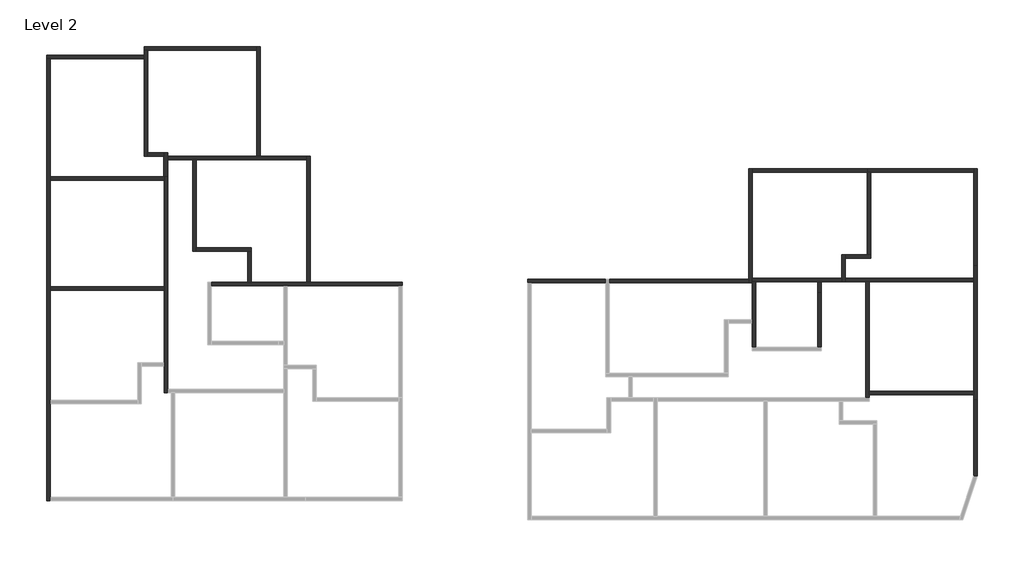
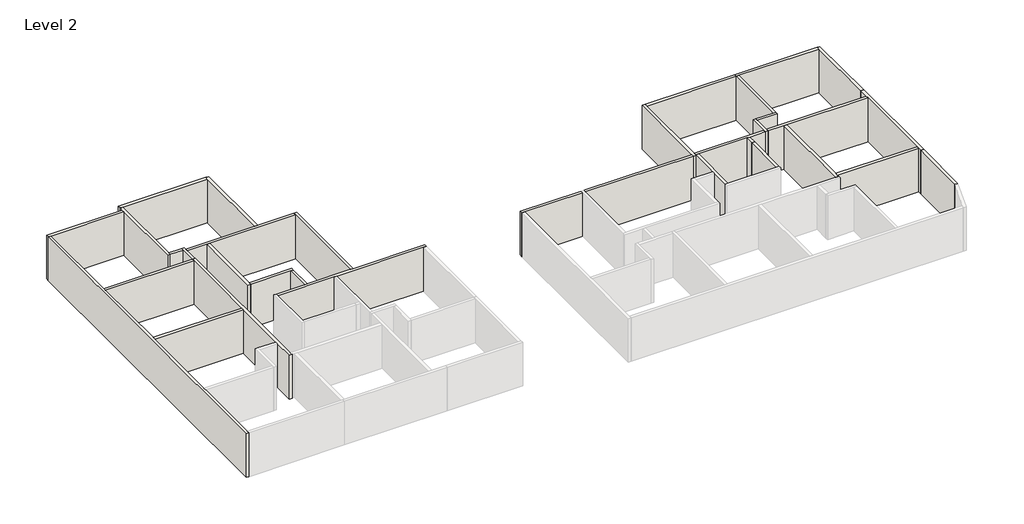
# One storey, part 2 of 2: 34 walls.
"""IFC4 building model written with IfcOpenShell, lengths in millimetres."""

from ifc_helpers import new_model, si_unit, frame, origin, place, context, project, spatial, polyline, outline, extrude, faceted_brep, element, save

model = new_model("IFC4")

# Units and contexts
model_context = context("Model", 3, world=origin())
ifc_project = project(units=[si_unit("LENGTHUNIT", "METRE", prefix="MILLI")], contexts=[model_context])

# Site, building, storey
site = spatial("IfcSite", under=ifc_project)
building = spatial("IfcBuilding", under=site)
storey = spatial("IfcBuildingStorey", under=building, Name="Level 2", Elevation=3000.0)

# Walls
placement = place(None, origin())
element("IfcWall", 1, ObjectType="Generic - 200mm", at=placement, inside=storey, context=model_context, shape_type="Brep", body=[
    faceted_brep([(24049.836337, 7619.475628, 3000.0), (24249.836337, 7619.475628, 3000.0), (30068.3425199, 7619.475628, 3000.0), (30068.3425199, 7619.475628, 6360.0), (24249.836337, 7619.475628, 6360.0), (24049.836337, 7619.475628, 6360.0), (24049.836337, 7819.475628, 3000.0), (24049.836337, 7819.475628, 6360.0), (30068.3425199, 7819.475628, 6360.0), (30068.3425199, 7819.475628, 3000.0)], [[[0, 1, 2, 3, 4, 5]], [[6, 7, 8, 9]], [[2, 1, 0, 6, 9]], [[5, 4, 3, 8, 7]], [[3, 2, 9, 8]], [[0, 5, 7, 6]]]),
])
element("IfcWall", 2, ObjectType="Generic - 200mm", at=placement, inside=storey, context=model_context, shape_type="Brep", body=[
    faceted_brep([(30068.3425199, 7819.475628, 3000.0), (30068.3425199, 7619.475628, 3000.0), (30068.3425199, 2319.475628, 3000.0), (30068.3425199, 2319.475628, 6360.0), (30068.3425199, 7619.475628, 6360.0), (30068.3425199, 7819.475628, 6360.0), (30268.3425199, 7819.475628, 3000.0), (30268.3425199, 7819.475628, 6360.0), (30268.3425199, 2319.475628, 6360.0), (30268.3425199, 2319.475628, 3000.0), (30117.9969803, 2319.475628, 3000.0), (30068.8612349, 2319.475628, 3000.0), (30068.8612349, 2319.475628, 6360.0)], [[[0, 1, 2, 3, 4, 5]], [[6, 7, 8, 9]], [[2, 1, 0, 6, 9, 10, 11]], [[3, 2, 11, 10, 9, 8, 12]], [[5, 4, 3, 12, 8, 7]], [[0, 5, 7, 6]]]),
])
element("IfcWall", 3, ObjectType="Generic - 200mm", at=placement, inside=storey, context=model_context, shape_type="Brep", body=[
    faceted_brep([(30068.8612349, 2319.475628, 3000.0), (30068.8612349, 1619.475628, 3000.0), (30068.8612349, 1419.475628, 3000.0), (30068.8612349, -4760.0098119, 3000.0), (30068.8612349, -4960.0098119, 3000.0), (30068.8612349, -5240.0098119, 3000.0), (30068.8612349, -5240.0098119, 6360.0), (30068.8612349, -4960.0098119, 6360.0), (30068.8612349, -4760.0098119, 6360.0), (30068.8612349, 1419.475628, 6360.0), (30068.8612349, 1619.475628, 6360.0), (30068.8612349, 2319.475628, 6360.0), (30268.8612349, 2319.475628, 3000.0), (30268.8612349, 2319.475628, 6360.0), (30268.8612349, -5240.0098119, 6360.0), (30268.8612349, -5240.0098119, 3000.0), (30118.5156953, 2319.475628, 3000.0), (30268.3425199, 2319.475628, 3000.0), (30118.5156953, -5240.0098119, 3000.0), (30069.3799498, -5240.0098119, 3000.0), (30069.3799498, -5240.0098119, 6360.0), (30268.3425199, 2319.475628, 6360.0)], [[[0, 1, 2, 3, 4, 5, 6, 7, 8, 9, 10, 11]], [[12, 13, 14, 15]], [[5, 4, 3, 2, 1, 0, 16, 17, 12, 15, 18, 19]], [[6, 5, 19, 18, 15, 14, 20]], [[11, 10, 9, 8, 7, 6, 20, 14, 13, 21]], [[0, 11, 21, 13, 12, 17, 16]]]),
])
element("IfcWall", 4, ObjectType="Generic - 200mm", at=placement, inside=storey, context=model_context, shape_type="Brep", body=[
    faceted_brep([(30069.3799498, -5240.0098119, 3000.0), (30069.3799498, -9543.0251929, 3000.0), (30069.3799498, -9543.0251929, 6360.0), (30069.3799498, -5240.0098119, 6360.0), (30269.3799498, -5240.0098119, 3000.0), (30269.3799498, -5240.0098119, 6360.0), (30269.3799498, -9575.863443, 6360.0), (30269.3799498, -9575.863443, 3000.0), (30119.0344102, -5240.0098119, 3000.0), (30268.8612349, -5240.0098119, 3000.0), (30268.8612349, -5240.0098119, 6360.0)], [[[0, 1, 2, 3]], [[4, 5, 6, 7]], [[1, 0, 8, 9, 4, 7]], [[3, 2, 6, 5, 10]], [[0, 3, 10, 5, 4, 9, 8]], [[2, 1, 7, 6]]]),
])
element("IfcWall", 5, ObjectType="Generic - 200mm", at=placement, inside=storey, context=model_context, shape_type="Brep", body=[
    faceted_brep([(24148.8612349, -5140.0098119, 3000.0), (24148.8612349, -4960.0098119, 3000.0), (24148.8612349, -4760.0098119, 3000.0), (24148.8612349, 1419.475628, 3000.0), (24148.8612349, 1419.475628, 6360.0), (24148.8612349, -4760.0098119, 6360.0), (24148.8612349, -4960.0098119, 6360.0), (24148.8612349, -5140.0098119, 6360.0), (23948.8612349, -5140.0098119, 3000.0), (23948.8612349, -5140.0098119, 6360.0), (23948.8612349, 1419.475628, 6360.0), (23948.8612349, 1419.475628, 3000.0)], [[[0, 1, 2, 3, 4, 5, 6, 7]], [[8, 9, 10, 11]], [[3, 2, 1, 0, 8, 11]], [[7, 6, 5, 4, 10, 9]], [[4, 3, 11, 10]], [[0, 7, 9, 8]]]),
])
element("IfcWall", 6, ObjectType="Generic - 200mm", at=placement, inside=storey, context=model_context, shape_type="Brep", body=[
    faceted_brep([(21249.836337, 799.475628, 3000.0), (21249.836337, -2276.2808257, 3000.0), (21249.836337, -2276.2808257, 6360.0), (21249.836337, 799.475628, 6360.0), (21449.836337, 799.475628, 3000.0), (21449.836337, 799.475628, 6360.0), (21449.836337, -2276.2808257, 6360.0), (21449.836337, -2276.2808257, 3000.0), (21299.4907974, 799.475628, 3000.0)], [[[0, 1, 2, 3]], [[4, 5, 6, 7]], [[1, 0, 8, 4, 7]], [[3, 2, 6, 5]], [[0, 3, 5, 4, 8]], [[2, 1, 7, 6]]]),
])
element("IfcWall", 7, ObjectType="Generic - 200mm", at=placement, inside=storey, context=model_context, shape_type="Brep", body=[
    faceted_brep([(17530.6041014, 1419.475628, 3000.0), (17530.6041014, -720.524372, 3000.0), (17530.6041014, -920.524372, 3000.0), (17530.6041014, -2276.2808257, 3000.0), (17530.6041014, -2276.2808257, 6360.0), (17530.6041014, -920.524372, 6360.0), (17530.6041014, -720.524372, 6360.0), (17530.6041014, 1419.475628, 6360.0), (17730.6041014, 1419.475628, 3000.0), (17730.6041014, 1419.475628, 6360.0), (17730.6041014, -2276.2808257, 6360.0), (17730.6041014, -2276.2808257, 3000.0)], [[[0, 1, 2, 3, 4, 5, 6, 7]], [[8, 9, 10, 11]], [[3, 2, 1, 0, 8, 11]], [[7, 6, 5, 4, 10, 9]], [[4, 3, 11, 10]], [[0, 7, 9, 8]]]),
])
element("IfcWall", 8, ObjectType="Generic - 200mm", at=placement, inside=storey, context=model_context, shape_type="Brep", body=[
    faceted_brep([(21449.836337, 799.475628, 3000.0), (21449.836337, 1419.475628, 3000.0), (21449.836337, 1419.475628, 6360.0), (21449.836337, 799.475628, 6360.0), (21249.836337, 799.475628, 3000.0), (21249.836337, 799.475628, 6360.0), (21249.836337, 1419.475628, 6360.0), (21249.836337, 1419.475628, 3000.0), (21299.4907974, 799.475628, 3000.0)], [[[0, 1, 2, 3]], [[4, 5, 6, 7]], [[1, 0, 8, 4, 7]], [[3, 2, 6, 5]], [[0, 3, 5, 4, 8]], [[2, 1, 7, 6]]]),
])
element("IfcWall", 9, ObjectType="Generic - 200mm", at=placement, inside=storey, context=model_context, shape_type="SweptSolid", body=[
    extrude(outline(polyline([(24049.836337, 7619.475628), (17528.8612349, 7619.475628), (17528.8612349, 7819.475628), (24049.836337, 7819.475628), (24049.836337, 7619.475628)])), frame((0.0, 0.0, 3000.0), z_axis=(0.0, 0.0, 1.0), x_axis=(1.0, 0.0, 0.0)), (0.0, 0.0, 1.0), 3360.0),
])
element("IfcWall", 10, ObjectType="Generic - 200mm", at=placement, inside=storey, context=model_context, shape_type="Brep", body=[
    faceted_brep([(22789.836337, 1419.475628, 3000.0), (22789.836337, 1619.475628, 3000.0), (22789.836337, 2754.475628, 3000.0), (22789.836337, 2954.475628, 3000.0), (22789.836337, 2954.475628, 6360.0), (22789.836337, 2754.475628, 6360.0), (22789.836337, 1619.475628, 6360.0), (22789.836337, 1419.475628, 6360.0), (22589.836337, 1419.475628, 3000.0), (22589.836337, 1419.475628, 6360.0), (22589.836337, 1619.475628, 6360.0), (22589.836337, 2954.475628, 6360.0), (22589.836337, 2954.475628, 3000.0), (22589.836337, 1619.475628, 3000.0)], [[[0, 1, 2, 3, 4, 5, 6, 7]], [[8, 9, 10, 11, 12, 13]], [[3, 2, 1, 0, 8, 13, 12]], [[7, 6, 5, 4, 11, 10, 9]], [[0, 7, 9, 8]], [[4, 3, 12, 11]]]),
])
element("IfcWall", 11, ObjectType="Generic - 200mm", at=placement, inside=storey, context=model_context, shape_type="Brep", body=[
    faceted_brep([(17328.8612349, 7819.475628, 3000.0), (17328.8612349, 1579.475628, 3000.0), (17328.8612349, 1379.475628, 3000.0), (17328.8612349, 1379.475628, 6360.0), (17328.8612349, 1579.475628, 6360.0), (17328.8612349, 7819.475628, 6360.0), (17528.8612349, 7819.475628, 3000.0), (17528.8612349, 7819.475628, 6360.0), (17528.8612349, 7619.475628, 6360.0), (17528.8612349, 1619.475628, 6360.0), (17528.8612349, 1419.475628, 6360.0), (17528.8612349, 1379.475628, 6360.0), (17528.8612349, 1379.475628, 3000.0), (17528.8612349, 1419.475628, 3000.0), (17528.8612349, 1619.475628, 3000.0), (17528.8612349, 7619.475628, 3000.0)], [[[0, 1, 2, 3, 4, 5]], [[6, 7, 8, 9, 10, 11, 12, 13, 14, 15]], [[2, 1, 0, 6, 15, 14, 13, 12]], [[5, 4, 3, 11, 10, 9, 8, 7]], [[0, 5, 7, 6]], [[3, 2, 12, 11]]]),
])
element("IfcWall", 12, ObjectType="Generic - 200mm", at=placement, inside=storey, context=model_context, shape_type="Brep", body=[
    faceted_brep([(22789.836337, 1419.475628, 3000.0), (23948.8612349, 1419.475628, 3000.0), (24148.8612349, 1419.475628, 3000.0), (30068.8612349, 1419.475628, 3000.0), (30068.8612349, 1419.475628, 6360.0), (24148.8612349, 1419.475628, 6360.0), (23948.8612349, 1419.475628, 6360.0), (22789.836337, 1419.475628, 6360.0), (22789.836337, 1619.475628, 3000.0), (22789.836337, 1619.475628, 6360.0), (30068.8612349, 1619.475628, 6360.0), (30068.8612349, 1619.475628, 3000.0)], [[[0, 1, 2, 3, 4, 5, 6, 7]], [[8, 9, 10, 11]], [[3, 2, 1, 0, 8, 11]], [[7, 6, 5, 4, 10, 9]], [[4, 3, 11, 10]], [[0, 7, 9, 8]]]),
])
element("IfcWall", 13, ObjectType="Generic - 200mm", at=placement, inside=storey, context=model_context, shape_type="SweptSolid", body=[
    extrude(outline(polyline([(9468.8612349, 1579.475628), (17328.8612349, 1579.475628), (17328.8612349, 1379.475628), (9468.8612349, 1379.475628), (9468.8612349, 1579.475628)])), frame((0.0, 0.0, 3000.0), z_axis=(0.0, 0.0, 1.0), x_axis=(1.0, 0.0, 0.0)), (0.0, 0.0, 1.0), 3360.0),
])
element("IfcWall", 14, ObjectType="Generic - 200mm", at=placement, inside=storey, context=model_context, shape_type="Brep", body=[
    faceted_brep([(22589.836337, 1619.475628, 3000.0), (17528.8612349, 1619.475628, 3000.0), (17528.8612349, 1619.475628, 6360.0), (22589.836337, 1619.475628, 6360.0), (22589.836337, 1419.475628, 3000.0), (22589.836337, 1419.475628, 6360.0), (21449.836337, 1419.475628, 6360.0), (21249.836337, 1419.475628, 6360.0), (17730.6041014, 1419.475628, 6360.0), (17530.6041014, 1419.475628, 6360.0), (17528.8612349, 1419.475628, 6360.0), (17528.8612349, 1419.475628, 3000.0), (17530.6041014, 1419.475628, 3000.0), (17730.6041014, 1419.475628, 3000.0), (21249.836337, 1419.475628, 3000.0), (21449.836337, 1419.475628, 3000.0)], [[[0, 1, 2, 3]], [[4, 5, 6, 7, 8, 9, 10, 11, 12, 13, 14, 15]], [[1, 0, 4, 15, 14, 13, 12, 11]], [[3, 2, 10, 9, 8, 7, 6, 5]], [[0, 3, 5, 4]], [[2, 1, 11, 10]]]),
])
element("IfcWall", 15, ObjectType="Generic - 200mm", at=placement, inside=storey, context=model_context, shape_type="Brep", body=[
    faceted_brep([(22789.836337, 2754.475628, 3000.0), (24249.836337, 2754.475628, 3000.0), (24249.836337, 2754.475628, 6360.0), (22789.836337, 2754.475628, 6360.0), (22789.836337, 2954.475628, 3000.0), (22789.836337, 2954.475628, 6360.0), (24049.836337, 2954.475628, 6360.0), (24249.836337, 2954.475628, 6360.0), (24249.836337, 2954.475628, 3000.0), (24049.836337, 2954.475628, 3000.0)], [[[0, 1, 2, 3]], [[4, 5, 6, 7, 8, 9]], [[1, 0, 4, 9, 8]], [[3, 2, 7, 6, 5]], [[2, 1, 8, 7]], [[0, 3, 5, 4]]]),
])
element("IfcWall", 16, ObjectType="Generic - 200mm", at=placement, inside=storey, context=model_context, shape_type="SweptSolid", body=[
    extrude(outline(polyline([(24249.836337, 7619.475628), (24249.836337, 2954.475628), (24049.836337, 2954.475628), (24049.836337, 7619.475628), (24249.836337, 7619.475628)])), frame((0.0, 0.0, 3000.0), z_axis=(0.0, 0.0, 1.0), x_axis=(1.0, 0.0, 0.0)), (0.0, 0.0, 1.0), 3360.0),
])
element("IfcWall", 17, ObjectType="Generic - 200mm", at=placement, inside=storey, context=model_context, shape_type="SweptSolid", body=[
    extrude(outline(polyline([(30068.8612349, -4960.0098119), (24148.8612349, -4960.0098119), (24148.8612349, -4760.0098119), (30068.8612349, -4760.0098119), (30068.8612349, -4960.0098119)])), frame((0.0, 0.0, 3000.0), z_axis=(0.0, 0.0, 1.0), x_axis=(1.0, 0.0, 0.0)), (0.0, 0.0, 1.0), 3360.0),
])
element("IfcWall", 18, ObjectType="Generic - 200mm", at=placement, inside=storey, context=model_context, shape_type="SweptSolid", body=[
    extrude(outline(polyline([(-15689.8304233, 949.8621849), (-22146.5113948, 949.8621849), (-22146.5113948, 1149.8621849), (-15689.8304233, 1149.8621849), (-15689.8304233, 949.8621849)])), frame((0.0, 0.0, 3000.0), z_axis=(0.0, 0.0, 1.0), x_axis=(1.0, 0.0, 0.0)), (0.0, 0.0, 1.0), 3360.0),
])
element("IfcWall", 19, ObjectType="Generic - 200mm", at=placement, inside=storey, context=model_context, shape_type="Brep", body=[
    faceted_brep([(-22146.5113948, -10959.6814279, 3000.0), (-22146.5113948, -10759.6814279, 3000.0), (-22146.5113948, -5479.1627129, 3000.0), (-22146.5113948, -5279.1627129, 3000.0), (-22146.5113948, 949.8621849, 3000.0), (-22146.5113948, 1149.8621849, 3000.0), (-22146.5113948, 7149.8621849, 3000.0), (-22146.5113948, 7349.8621849, 3000.0), (-22146.5113948, 14029.8621849, 3000.0), (-22146.5113948, 14029.8621849, 6360.0), (-22146.5113948, 7349.8621849, 6360.0), (-22146.5113948, 7149.8621849, 6360.0), (-22146.5113948, 1149.8621849, 6360.0), (-22146.5113948, 949.8621849, 6360.0), (-22146.5113948, -5279.1627129, 6360.0), (-22146.5113948, -5479.1627129, 6360.0), (-22146.5113948, -10759.6814279, 6360.0), (-22146.5113948, -10959.6814279, 6360.0), (-22346.5113948, -10959.6814279, 3000.0), (-22346.5113948, -10959.6814279, 6360.0), (-22346.5113948, 14029.8621849, 6360.0), (-22346.5113948, 14029.8621849, 3000.0)], [[[0, 1, 2, 3, 4, 5, 6, 7, 8, 9, 10, 11, 12, 13, 14, 15, 16, 17]], [[18, 19, 20, 21]], [[8, 7, 6, 5, 4, 3, 2, 1, 0, 18, 21]], [[17, 16, 15, 14, 13, 12, 11, 10, 9, 20, 19]], [[9, 8, 21, 20]], [[0, 17, 19, 18]]]),
])
element("IfcWall", 20, ObjectType="Generic - 200mm", at=placement, inside=storey, context=model_context, shape_type="Brep", body=[
    faceted_brep([(-15689.8304233, 7349.8621849, 3000.0), (-15709.8304233, 7349.8621849, 3000.0), (-22146.5113948, 7349.8621849, 3000.0), (-22146.5113948, 7349.8621849, 6360.0), (-15709.8304233, 7349.8621849, 6360.0), (-15689.8304233, 7349.8621849, 6360.0), (-15689.8304233, 7149.8621849, 3000.0), (-15689.8304233, 7149.8621849, 6360.0), (-22146.5113948, 7149.8621849, 6360.0), (-22146.5113948, 7149.8621849, 3000.0)], [[[0, 1, 2, 3, 4, 5]], [[6, 7, 8, 9]], [[2, 1, 0, 6, 9]], [[5, 4, 3, 8, 7]], [[3, 2, 9, 8]], [[0, 5, 7, 6]]]),
])
element("IfcWall", 21, ObjectType="Generic - 200mm", at=placement, inside=storey, context=model_context, shape_type="Brep", body=[
    faceted_brep([(-15489.8304233, -4853.7013134, 3000.0), (-15489.8304233, -4839.1627129, 3000.0), (-15489.8304233, -4639.1627129, 3000.0), (-15489.8304233, 7349.8621849, 3000.0), (-15489.8304233, 7349.8621849, 6360.0), (-15489.8304233, -4639.1627129, 6360.0), (-15489.8304233, -4839.1627129, 6360.0), (-15489.8304233, -4853.7013134, 6360.0), (-15689.8304233, -4853.7013134, 3000.0), (-15689.8304233, -4853.7013134, 6360.0), (-15689.8304233, -3359.1627129, 6360.0), (-15689.8304233, -3159.1627129, 6360.0), (-15689.8304233, 949.8621849, 6360.0), (-15689.8304233, 1149.8621849, 6360.0), (-15689.8304233, 7149.8621849, 6360.0), (-15689.8304233, 7349.8621849, 6360.0), (-15689.8304233, 7349.8621849, 3000.0), (-15689.8304233, 7149.8621849, 3000.0), (-15689.8304233, 1149.8621849, 3000.0), (-15689.8304233, 949.8621849, 3000.0), (-15689.8304233, -3159.1627129, 3000.0), (-15689.8304233, -3359.1627129, 3000.0), (-15509.8304233, 7349.8621849, 3000.0), (-15509.8304233, 7349.8621849, 6360.0)], [[[0, 1, 2, 3, 4, 5, 6, 7]], [[8, 9, 10, 11, 12, 13, 14, 15, 16, 17, 18, 19, 20, 21]], [[3, 2, 1, 0, 8, 21, 20, 19, 18, 17, 16, 22]], [[7, 6, 5, 4, 23, 15, 14, 13, 12, 11, 10, 9]], [[0, 7, 9, 8]], [[4, 3, 22, 16, 15, 23]]]),
])
element("IfcWall", 22, ObjectType="Generic - 200mm", at=placement, inside=storey, context=model_context, shape_type="Brep", body=[
    faceted_brep([(-16829.8304233, 14229.8621849, 3000.0), (-22346.5113948, 14229.8621849, 3000.0), (-22346.5113948, 14229.8621849, 6360.0), (-16829.8304233, 14229.8621849, 6360.0), (-16829.8304233, 14029.8621849, 3000.0), (-16829.8304233, 14029.8621849, 6360.0), (-22146.5113948, 14029.8621849, 6360.0), (-22346.5113948, 14029.8621849, 6360.0), (-22346.5113948, 14029.8621849, 3000.0), (-22146.5113948, 14029.8621849, 3000.0)], [[[0, 1, 2, 3]], [[4, 5, 6, 7, 8, 9]], [[1, 0, 4, 9, 8]], [[3, 2, 7, 6, 5]], [[2, 1, 8, 7]], [[0, 3, 5, 4]]]),
])
element("IfcWall", 23, ObjectType="Generic - 200mm", at=placement, inside=storey, context=model_context, shape_type="Brep", body=[
    faceted_brep([(-14089.8304233, 8320.8372871, 3000.0), (-14089.8304233, 3139.0944206, 3000.0), (-14089.8304233, 3139.0944206, 6360.0), (-14089.8304233, 8320.8372871, 6360.0), (-13889.8304233, 8320.8372871, 3000.0), (-13889.8304233, 8320.8372871, 6360.0), (-13889.8304233, 3339.0944206, 6360.0), (-13889.8304233, 3139.0944206, 6360.0), (-13889.8304233, 3139.0944206, 3000.0), (-13889.8304233, 3339.0944206, 3000.0)], [[[0, 1, 2, 3]], [[4, 5, 6, 7, 8, 9]], [[1, 0, 4, 9, 8]], [[3, 2, 7, 6, 5]], [[2, 1, 8, 7]], [[0, 3, 5, 4]]]),
])
element("IfcWall", 24, ObjectType="Generic - 200mm", at=placement, inside=storey, context=model_context, shape_type="Brep", body=[
    faceted_brep([(-13889.8304233, 3139.0944206, 3000.0), (-10970.3449834, 3139.0944206, 3000.0), (-10770.3449834, 3139.0944206, 3000.0), (-10770.3449834, 3139.0944206, 6360.0), (-10970.3449834, 3139.0944206, 6360.0), (-13889.8304233, 3139.0944206, 6360.0), (-13889.8304233, 3339.0944206, 3000.0), (-13889.8304233, 3339.0944206, 6360.0), (-10770.3449834, 3339.0944206, 6360.0), (-10770.3449834, 3339.0944206, 3000.0)], [[[0, 1, 2, 3, 4, 5]], [[6, 7, 8, 9]], [[2, 1, 0, 6, 9]], [[5, 4, 3, 8, 7]], [[0, 5, 7, 6]], [[3, 2, 9, 8]]]),
])
element("IfcWall", 25, ObjectType="Generic - 200mm", at=placement, inside=storey, context=model_context, shape_type="SweptSolid", body=[
    extrude(outline(polyline([(-10970.3449834, 1400.8372871), (-10970.3449834, 3139.0944206), (-10770.3449834, 3139.0944206), (-10770.3449834, 1400.8372871), (-10970.3449834, 1400.8372871)])), frame((0.0, 0.0, 3000.0), z_axis=(0.0, 0.0, 1.0), x_axis=(1.0, 0.0, 0.0)), (0.0, 0.0, 1.0), 3360.0),
])
element("IfcWall", 26, ObjectType="Generic - 200mm", at=placement, inside=storey, context=model_context, shape_type="Brep", body=[
    faceted_brep([(-2230.3449834, 1400.8372871, 3000.0), (-7430.3449834, 1400.8372871, 3000.0), (-7630.3449834, 1400.8372871, 3000.0), (-10770.3449834, 1400.8372871, 3000.0), (-10970.3449834, 1400.8372871, 3000.0), (-13026.101437, 1400.8372871, 3000.0), (-13026.101437, 1400.8372871, 6360.0), (-10970.3449834, 1400.8372871, 6360.0), (-10770.3449834, 1400.8372871, 6360.0), (-7630.3449834, 1400.8372871, 6360.0), (-7430.3449834, 1400.8372871, 6360.0), (-2230.3449834, 1400.8372871, 6360.0), (-2230.3449834, 1200.8372871, 3000.0), (-2230.3449834, 1200.8372871, 6360.0), (-2430.3449834, 1200.8372871, 6360.0), (-8730.3449834, 1200.8372871, 6360.0), (-8930.3449834, 1200.8372871, 6360.0), (-13026.101437, 1200.8372871, 6360.0), (-13026.101437, 1200.8372871, 3000.0), (-8930.3449834, 1200.8372871, 3000.0), (-8730.3449834, 1200.8372871, 3000.0), (-2430.3449834, 1200.8372871, 3000.0)], [[[0, 1, 2, 3, 4, 5, 6, 7, 8, 9, 10, 11]], [[12, 13, 14, 15, 16, 17, 18, 19, 20, 21]], [[5, 4, 3, 2, 1, 0, 12, 21, 20, 19, 18]], [[11, 10, 9, 8, 7, 6, 17, 16, 15, 14, 13]], [[0, 11, 13, 12]], [[6, 5, 18, 17]]]),
])
element("IfcWall", 27, ObjectType="Generic - 200mm", at=placement, inside=storey, context=model_context, shape_type="Brep", body=[
    faceted_brep([(-7430.3449834, 1400.8372871, 3000.0), (-7430.3449834, 8520.8372871, 3000.0), (-7430.3449834, 8520.8372871, 6360.0), (-7430.3449834, 1400.8372871, 6360.0), (-7630.3449834, 1400.8372871, 3000.0), (-7630.3449834, 1400.8372871, 6360.0), (-7630.3449834, 8320.8372871, 6360.0), (-7630.3449834, 8520.8372871, 6360.0), (-7630.3449834, 8520.8372871, 3000.0), (-7630.3449834, 8320.8372871, 3000.0)], [[[0, 1, 2, 3]], [[4, 5, 6, 7, 8, 9]], [[1, 0, 4, 9, 8]], [[3, 2, 7, 6, 5]], [[0, 3, 5, 4]], [[2, 1, 8, 7]]]),
])
element("IfcWall", 28, ObjectType="Generic - 200mm", at=placement, inside=storey, context=model_context, shape_type="Brep", body=[
    faceted_brep([(-7630.3449834, 8520.8372871, 3000.0), (-10270.3449834, 8520.8372871, 3000.0), (-10470.3449834, 8520.8372871, 3000.0), (-15509.8304233, 8520.8372871, 3000.0), (-15509.8304233, 8520.8372871, 6360.0), (-10470.3449834, 8520.8372871, 6360.0), (-10270.3449834, 8520.8372871, 6360.0), (-7630.3449834, 8520.8372871, 6360.0), (-7630.3449834, 8320.8372871, 3000.0), (-7630.3449834, 8320.8372871, 6360.0), (-13889.8304233, 8320.8372871, 6360.0), (-14089.8304233, 8320.8372871, 6360.0), (-15509.8304233, 8320.8372871, 6360.0), (-15509.8304233, 8320.8372871, 3000.0), (-14089.8304233, 8320.8372871, 3000.0), (-13889.8304233, 8320.8372871, 3000.0)], [[[0, 1, 2, 3, 4, 5, 6, 7]], [[8, 9, 10, 11, 12, 13, 14, 15]], [[3, 2, 1, 0, 8, 15, 14, 13]], [[7, 6, 5, 4, 12, 11, 10, 9]], [[0, 7, 9, 8]], [[4, 3, 13, 12]]]),
])
element("IfcWall", 29, ObjectType="Generic - 200mm", at=placement, inside=storey, context=model_context, shape_type="Brep", body=[
    faceted_brep([(-16629.8304233, 8515.8372871, 3000.0), (-16629.8304233, 8715.8372871, 3000.0), (-16629.8304233, 14520.8372871, 3000.0), (-16629.8304233, 14520.8372871, 6360.0), (-16629.8304233, 8715.8372871, 6360.0), (-16629.8304233, 8515.8372871, 6360.0), (-16829.8304233, 8515.8372871, 3000.0), (-16829.8304233, 8515.8372871, 6360.0), (-16829.8304233, 14029.8621849, 6360.0), (-16829.8304233, 14229.8621849, 6360.0), (-16829.8304233, 14520.8372871, 6360.0), (-16829.8304233, 14520.8372871, 3000.0), (-16829.8304233, 14229.8621849, 3000.0), (-16829.8304233, 14029.8621849, 3000.0)], [[[0, 1, 2, 3, 4, 5]], [[6, 7, 8, 9, 10, 11, 12, 13]], [[2, 1, 0, 6, 13, 12, 11]], [[5, 4, 3, 10, 9, 8, 7]], [[0, 5, 7, 6]], [[3, 2, 11, 10]]]),
])
element("IfcWall", 30, ObjectType="Generic - 200mm", at=placement, inside=storey, context=model_context, shape_type="Brep", body=[
    faceted_brep([(9268.8612349, 1579.9901881, 3000.0), (4843.716007, 1579.9901881, 3000.0), (4843.716007, 1579.9901881, 6360.0), (9268.8612349, 1579.9901881, 6360.0), (9268.8612349, 1379.9901881, 3000.0), (9268.8612349, 1379.9901881, 6360.0), (5043.716007, 1379.9901881, 6360.0), (4843.716007, 1379.9901881, 6360.0), (4843.716007, 1379.9901881, 3000.0), (5043.716007, 1379.9901881, 3000.0)], [[[0, 1, 2, 3]], [[4, 5, 6, 7, 8, 9]], [[1, 0, 4, 9, 8]], [[3, 2, 7, 6, 5]], [[2, 1, 8, 7]], [[0, 3, 5, 4]]]),
])
element("IfcWall", 31, ObjectType="Generic - 200mm", at=placement, inside=storey, context=model_context, shape_type="Brep", body=[
    faceted_brep([(-10270.3449834, 8520.8372871, 3000.0), (-10270.3449834, 14720.8372871, 3000.0), (-10270.3449834, 14720.8372871, 6360.0), (-10270.3449834, 8520.8372871, 6360.0), (-10470.3449834, 8520.8372871, 3000.0), (-10470.3449834, 8520.8372871, 6360.0), (-10470.3449834, 14520.8372871, 6360.0), (-10470.3449834, 14720.8372871, 6360.0), (-10470.3449834, 14720.8372871, 3000.0), (-10470.3449834, 14520.8372871, 3000.0)], [[[0, 1, 2, 3]], [[4, 5, 6, 7, 8, 9]], [[1, 0, 4, 9, 8]], [[3, 2, 7, 6, 5]], [[0, 3, 5, 4]], [[2, 1, 8, 7]]]),
])
element("IfcWall", 32, ObjectType="Generic - 200mm", at=placement, inside=storey, context=model_context, shape_type="Brep", body=[
    faceted_brep([(-10470.3449834, 14720.8372871, 3000.0), (-16829.8304233, 14720.8372871, 3000.0), (-16829.8304233, 14720.8372871, 6360.0), (-10470.3449834, 14720.8372871, 6360.0), (-10470.3449834, 14520.8372871, 3000.0), (-10470.3449834, 14520.8372871, 6360.0), (-16629.8304233, 14520.8372871, 6360.0), (-16829.8304233, 14520.8372871, 6360.0), (-16829.8304233, 14520.8372871, 3000.0), (-16629.8304233, 14520.8372871, 3000.0)], [[[0, 1, 2, 3]], [[4, 5, 6, 7, 8, 9]], [[1, 0, 4, 9, 8]], [[3, 2, 7, 6, 5]], [[0, 3, 5, 4]], [[2, 1, 8, 7]]]),
])
element("IfcWall", 33, ObjectType="Generic - 200mm", at=placement, inside=storey, context=model_context, shape_type="Brep", body=[
    faceted_brep([(-15709.8304233, 8715.8372871, 3000.0), (-15709.8304233, 8515.8372871, 3000.0), (-15709.8304233, 7349.8621849, 3000.0), (-15709.8304233, 7349.8621849, 6360.0), (-15709.8304233, 8515.8372871, 6360.0), (-15709.8304233, 8715.8372871, 6360.0), (-15509.8304233, 8715.8372871, 3000.0), (-15509.8304233, 8715.8372871, 6360.0), (-15509.8304233, 8520.8372871, 6360.0), (-15509.8304233, 8320.8372871, 6360.0), (-15509.8304233, 7349.8621849, 6360.0), (-15509.8304233, 7349.8621849, 3000.0), (-15509.8304233, 8320.8372871, 3000.0), (-15509.8304233, 8520.8372871, 3000.0), (-15689.8304233, 7349.8621849, 3000.0), (-15689.8304233, 7349.8621849, 6360.0)], [[[0, 1, 2, 3, 4, 5]], [[6, 7, 8, 9, 10, 11, 12, 13]], [[2, 1, 0, 6, 13, 12, 11, 14]], [[5, 4, 3, 15, 10, 9, 8, 7]], [[3, 2, 14, 11, 10, 15]], [[0, 5, 7, 6]]]),
])
element("IfcWall", 34, ObjectType="Generic - 200mm", at=placement, inside=storey, context=model_context, shape_type="SweptSolid", body=[
    extrude(outline(polyline([(-15709.8304233, 8515.8372871), (-16629.8304233, 8515.8372871), (-16629.8304233, 8715.8372871), (-15709.8304233, 8715.8372871), (-15709.8304233, 8515.8372871)])), frame((0.0, 0.0, 3000.0), z_axis=(0.0, 0.0, 1.0), x_axis=(1.0, 0.0, 0.0)), (0.0, 0.0, 1.0), 3360.0),
])

save(model, "model.ifc")

# Revit data of these elements
# Type "Generic - 200mm"
#   Layers, outside or top first: 20 cm no material (function 1)
# Elements 1, 2, 3, 4, 5, 6, 7, 8, 9, 10, 11, 12, 13, 14, 15, 16, 17, 18, 19, 20, 21, 22, 23, 24, 25, 26, 27, 28, 29, 30, 31, 32, 33, 34 (IfcWall, "Generic - 200mm")
#   Top Offset = 0 cm
#   Base Offset = 0 cm
#   wall height = 336 cm
#   Phase Created = New Construction
#   Base Constraint = Level 2
#   Top Constraint = Level 3
#   Materials on its faces: "Default Wall"
# Materials
#   "Default Wall": class "Miscellaneous", colour RGB 128 128 128, transparency 0, Cost = 0
